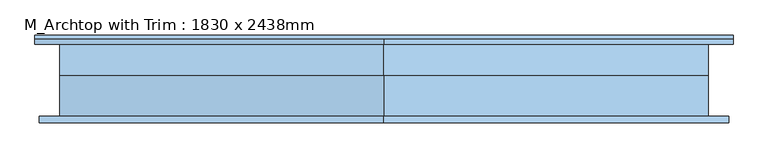
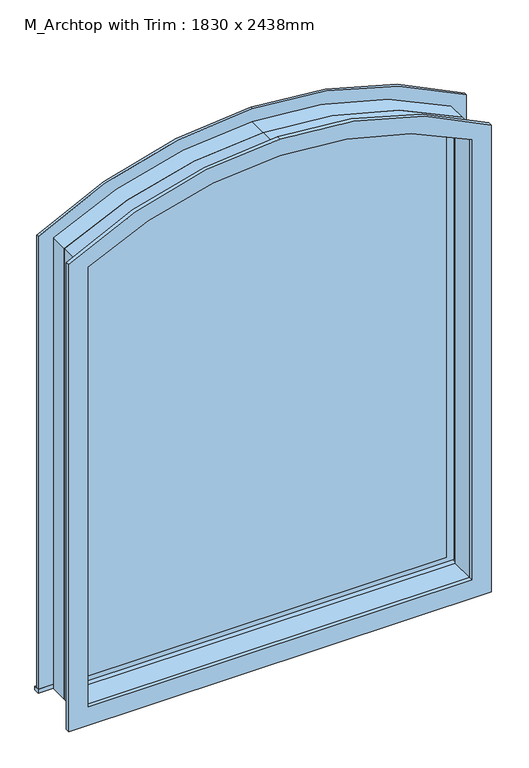
"""IFC4 building model written with IfcOpenShell, lengths in millimetres: window geometry, M_Archtop with Trim : 1830 x 2438mm."""

from ifc_helpers import new_model, si_unit, point, frame, frame_2d, origin, place, context, project, spatial, polyline, circle_curve, trimmed, segment, composite_curve, outline, extrude, source, transform, mapped, element, save


def m_archtop_with_trim_1830_x_2438mm_7157e706(model_context):
    return source(origin(), model_context, "Body", "SweptSolid", [
        extrude(outline(composite_curve([segment(polyline([(336.75, 903.8802979), (2486.7895349, 903.8802979)]), True, "CONTINUOUS"), segment(trimmed(circle_curve(frame_2d((913.0, 7.9302979)), 1810.95), [point((2486.7895349, 903.8802979))], [point((2723.95, 7.9302979))], False, "CARTESIAN"), True, "CONTINUOUS"), segment(trimmed(circle_curve(frame_2d((913.0, 7.9302979)), 1810.95), [point((2723.95, 7.9302979))], [point((2486.7895349, -888.019702))], False, "CARTESIAN"), True, "CONTINUOUS"), segment(polyline([(2486.7895349, -888.019702), (336.75, -888.019702), (336.75, 903.8802979)]), True, "CONTINUOUS")], self_intersect=False), holes=[composite_curve([segment(polyline([(368.5, 859.4302979), (368.5, -843.5697021), (2464.3533948, -843.5697021)]), True, "CONTINUOUS"), segment(trimmed(circle_curve(frame_2d((913.0, 7.9302979)), 1769.675), [point((2464.3533948, -843.5697021))], [point((2682.675, 7.9302979))], True, "CARTESIAN"), True, "CONTINUOUS"), segment(trimmed(circle_curve(frame_2d((913.0, 7.9302979)), 1769.675), [point((2682.675, 7.9302979))], [point((2464.3533948, 859.4302979))], True, "CARTESIAN"), True, "CONTINUOUS"), segment(polyline([(2464.3533948, 859.4302979), (368.5, 859.4302979)]), True, "CONTINUOUS")], self_intersect=False)]), frame((0.0, 38.1, 0.0), z_axis=(0.0, 1.0, 0.0), x_axis=(0.0, 0.0, 1.0)), (0.0, 0.0, 1.0), 44.45),
        extrude(outline(polyline([(-972.9697019, 127.3), (996.930298, 127.3), (996.930298, 101.6), (-972.9697019, 101.6), (-972.9697019, 127.3)])), frame((0.0, 0.0, 305.0), z_axis=(0.0, 0.0, 1.0), x_axis=(1.0, 0.0, 0.0)), (0.0, 0.0, 1.0), 19.05),
        extrude(outline(composite_curve([segment(polyline([(324.05, 907.9302979), (324.05, 996.930298), (2527.9180866, 996.930298)]), True, "CONTINUOUS"), segment(trimmed(circle_curve(frame_2d((913.0, 11.980298)), 1891.5831805), [point((2527.9180866, 996.930298))], [point((2804.5831805, 11.980298))], False, "CARTESIAN"), True, "CONTINUOUS"), segment(trimmed(circle_curve(frame_2d((913.0, 11.980298)), 1891.5831805), [point((2804.5831805, 11.980298))], [point((2527.9180866, -972.9697019))], False, "CARTESIAN"), True, "CONTINUOUS"), segment(polyline([(2527.9180866, -972.9697019), (324.05, -972.9697019), (324.05, -883.969702), (2486.7895348, -883.969702)]), True, "CONTINUOUS"), segment(trimmed(circle_curve(frame_2d((913.0, 11.980298)), 1810.95), [point((2486.7895348, -883.969702))], [point((2723.95, 11.980298))], True, "CARTESIAN"), True, "CONTINUOUS"), segment(trimmed(circle_curve(frame_2d((913.0, 11.980298)), 1810.95), [point((2723.95, 11.980298))], [point((2486.7895349, 907.9302979))], True, "CARTESIAN"), True, "CONTINUOUS"), segment(polyline([(2486.7895349, 907.9302979), (324.05, 907.9302979)]), True, "CONTINUOUS")], self_intersect=False)), frame((0.0, 101.6, 0.0), z_axis=(0.0, 1.0, 0.0), x_axis=(0.0, 0.0, 1.0)), (0.0, 0.0, 1.0), 13.0),
        extrude(outline(composite_curve([segment(polyline([(247.75, -960.269702), (247.75, 984.2302979), (2520.8214166, 984.2302979)]), True, "CONTINUOUS"), segment(trimmed(circle_curve(frame_2d((913.0, 11.980298)), 1878.9251635), [point((2520.8214166, 984.2302979))], [point((2791.9251635, 11.980298))], False, "CARTESIAN"), True, "CONTINUOUS"), segment(trimmed(circle_curve(frame_2d((913.0, 11.980298)), 1878.9251635), [point((2791.9251635, 11.980298))], [point((2520.8214165, -960.269702))], False, "CARTESIAN"), True, "CONTINUOUS"), segment(polyline([(2520.8214165, -960.269702), (247.75, -960.269702)]), True, "CONTINUOUS")], self_intersect=False), holes=[composite_curve([segment(polyline([(336.75, -871.2697029), (2479.3883613, -871.2697029)]), True, "CONTINUOUS"), segment(trimmed(circle_curve(frame_2d((913.0, 11.980298)), 1798.25), [point((2479.3883613, -871.2697029))], [point((2711.25, 11.980298))], True, "CARTESIAN"), True, "CONTINUOUS"), segment(trimmed(circle_curve(frame_2d((913.0000002, 11.980298)), 1798.2499998), [point((2711.25, 11.980298))], [point((2479.3883613, 895.2302988))], True, "CARTESIAN"), True, "CONTINUOUS"), segment(polyline([(2479.3883613, 895.2302988), (336.75, 895.2302988), (336.75, -871.2697029)]), True, "CONTINUOUS")], self_intersect=False)]), frame((0.0, -120.6, 0.0), z_axis=(0.0, 1.0, 0.0), x_axis=(0.0, 0.0, 1.0)), (0.0, 0.0, 1.0), 19.0),
        extrude(outline(composite_curve([segment(polyline([(368.5, -839.519702), (368.5, 863.4802977), (2464.6545931, 863.4802977)]), True, "CONTINUOUS"), segment(trimmed(circle_curve(frame_2d((913.0, 11.980298)), 1769.9390458), [point((2464.6545931, 863.4802977))], [point((2682.9390458, 11.980298))], False, "CARTESIAN"), True, "CONTINUOUS"), segment(trimmed(circle_curve(frame_2d((913.0, 11.980298)), 1769.9390458), [point((2682.9390458, 11.980298))], [point((2464.6545929, -839.519702))], False, "CARTESIAN"), True, "CONTINUOUS"), segment(polyline([(2464.6545929, -839.519702), (368.5, -839.519702)]), True, "CONTINUOUS")], self_intersect=False)), frame((0.0, 28.575, 0.0), z_axis=(0.0, 1.0, 0.0), x_axis=(0.0, 0.0, 1.0)), (0.0, 0.0, 1.0), 12.7),
        extrude(outline(composite_curve([segment(polyline([(305.0, 926.980298), (2497.8264889, 926.980298)]), True, "CONTINUOUS"), segment(trimmed(circle_curve(frame_2d((913.0, 11.980298)), 1830.0), [point((2497.8264889, 926.980298))], [point((2743.0, 11.980298))], False, "CARTESIAN"), True, "CONTINUOUS"), segment(trimmed(circle_curve(frame_2d((913.0, 11.980298)), 1830.0), [point((2743.0, 11.980298))], [point((2497.8264889, -903.019702))], False, "CARTESIAN"), True, "CONTINUOUS"), segment(polyline([(2497.8264889, -903.019702), (305.0, -903.019702), (305.0, 926.980298)]), True, "CONTINUOUS")], self_intersect=False), holes=[composite_curve([segment(polyline([(336.75, 895.2302988), (336.75, -871.269702), (2482.779909, -871.269702)]), True, "CONTINUOUS"), segment(trimmed(circle_curve(frame_2d((913.0, 11.980298)), 1801.2050203), [point((2482.779909, -871.269702))], [point((2714.2050203, 11.980298))], True, "CARTESIAN"), True, "CONTINUOUS"), segment(trimmed(circle_curve(frame_2d((913.0, 11.980298)), 1801.2050203), [point((2714.2050203, 11.980298))], [point((2482.7799085, 895.2302988))], True, "CARTESIAN"), True, "CONTINUOUS"), segment(polyline([(2482.7799085, 895.2302988), (336.75, 895.2302988)]), True, "CONTINUOUS")], self_intersect=False)]), frame((0.0, -101.6, 0.0), z_axis=(0.0, 1.0, 0.0), x_axis=(0.0, 0.0, 1.0)), (0.0, 0.0, 1.0), 114.3),
        extrude(outline(composite_curve([segment(polyline([(305.0, -903.019702), (305.0, 926.980298), (2497.8264889, 926.980298)]), True, "CONTINUOUS"), segment(trimmed(circle_curve(frame_2d((913.0, 11.980298)), 1830.0), [point((2497.8264889, 926.980298))], [point((2743.0, 11.980298))], False, "CARTESIAN"), True, "CONTINUOUS"), segment(trimmed(circle_curve(frame_2d((913.0, 11.980298)), 1830.0), [point((2743.0, 11.980298))], [point((2497.8264889, -903.019702))], False, "CARTESIAN"), True, "CONTINUOUS"), segment(polyline([(2497.8264889, -903.019702), (305.0, -903.019702)]), True, "CONTINUOUS")], self_intersect=False), holes=[composite_curve([segment(polyline([(324.05, -883.969702), (2488.8332662, -883.969702)]), True, "CONTINUOUS"), segment(trimmed(circle_curve(frame_2d((913.0, 11.980298)), 1812.726368), [point((2488.8332662, -883.969702))], [point((2725.726368, 11.980298))], True, "CARTESIAN"), True, "CONTINUOUS"), segment(trimmed(circle_curve(frame_2d((913.0, 11.980298)), 1812.726368), [point((2725.726368, 11.980298))], [point((2488.8332662, 907.930298))], True, "CARTESIAN"), True, "CONTINUOUS"), segment(polyline([(2488.8332662, 907.930298), (324.05, 907.930298), (324.05, -883.969702)]), True, "CONTINUOUS")], self_intersect=False)]), frame((0.0, 12.7, 0.0), z_axis=(0.0, 1.0, 0.0), x_axis=(0.0, 0.0, 1.0)), (0.0, 0.0, 1.0), 88.9),
    ])


if __name__ == "__main__":
    model = new_model("IFC4")
    model_context = context("Model", 3, world=origin())
    ifc_project = project(units=[si_unit("LENGTHUNIT", "METRE", prefix="MILLI")], contexts=[model_context])
    site = spatial("IfcSite", under=ifc_project)
    building = spatial("IfcBuilding", under=site)
    placement = place(None, origin())
    m_archtop_with_trim_1830_x_2438mm_shape = m_archtop_with_trim_1830_x_2438mm_7157e706(model_context)
    element("IfcWindow", 1, ObjectType="M_Archtop with Trim : 1830 x 2438mm", at=placement, inside=building, context=model_context, shape_type="MappedRepresentation", body=[
        mapped(m_archtop_with_trim_1830_x_2438mm_shape, transform((0.0, 0.0, 0.0), x_axis=(1.0, 0.0, 0.0), y_axis=(0.0, 1.0, 0.0), z_axis=(0.0, 0.0, 1.0))),
    ])
    save(model, "model.ifc")

# Revit data of these elements
# Type "M_Archtop with Trim : 1830 x 2438mm"
#   Type Mark = "16"
#   Construction Type Id = "GSP4R"
#   Analytic Construction = "1/8 in Pilkington single glazing"
#   Visual Light Transmittance = 0.9
#   Solar Heat Gain Coefficient = 0.78
#   Heat Transfer Coefficient (U) = 3.6886 W/(m²·K)
#   Height = 7' - 11.98425"
#   Radius = 6' - 0.04724"
#   Default Sill Height = 1' - 0.00787"
#   Trim Projection - Ext. = 0' - 0.51181"
#   Trim Projection - Int. = 0' - 0.74803"
#   Trim Width - Exterior = 0' - 3.50394"
#   Trim Width - Interior = 0' - 3.50394"
#   Width = 6' - 0.04724"
#   Glass Pane Material = Glass
#   Sash = Sash
#   Trim Exterior Material = Trim
#   Trim Interior Material = Trim
#   Wall Closure = (empty or 0)
# Element 1 (IfcWindow, "M_Archtop with Trim : 1830 x 2438mm")
#   Materials on its faces: "Trim", "Sash", "Glass"
# Materials
#   "Glass": class "Glass", colour RGB 0 128 192, transparency 0.75, Description = "Soda Lime Glass", Cost = 0
#   "Sash": class "Wood", colour RGB 224 178 126, transparency 0, Cost = 0
#   "Trim": class "Wood", colour RGB 224 178 126, transparency 0
